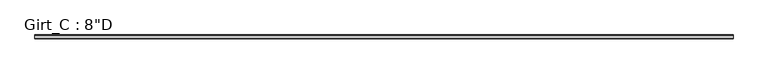
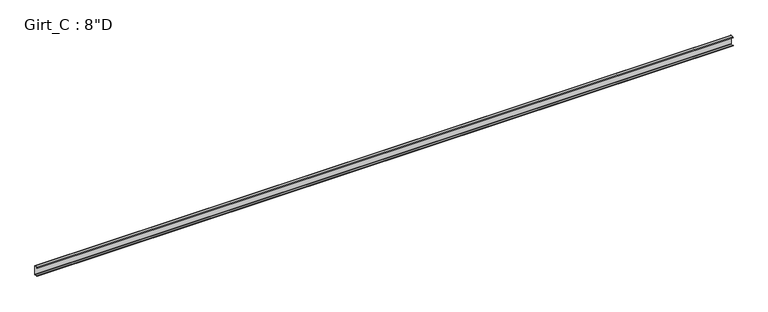
"""IFC4 building model written with IfcOpenShell, lengths in millimetres: beam geometry."""

from ifc_helpers import new_model, si_unit, point, frame, frame_2d, origin, place, context, project, spatial, polyline, circle_curve, trimmed, segment, composite_curve, outline, extrude, source, transform, mapped, element, save


def beam_3230b69d(model_context):
    return source(origin(), model_context, "Body", "SweptSolid", [
        extrude(outline(composite_curve([segment(polyline([(-63.5, 101.6), (-3.3734375, 101.6)]), True, "CONTINUOUS"), segment(trimmed(circle_curve(frame_2d((-3.3734375, 96.8375)), 4.7625), [point((-3.3734375, 101.6))], [point((1.3890625, 96.8375))], False, "CARTESIAN"), True, "CONTINUOUS"), segment(polyline([(1.3890625, 96.8375), (1.3890625, -96.8375)]), True, "CONTINUOUS"), segment(trimmed(circle_curve(frame_2d((-3.3734375, -96.8375)), 4.7625), [point((1.3890625, -96.8375))], [point((-3.3734375, -101.6))], False, "CARTESIAN"), True, "CONTINUOUS"), segment(polyline([(-3.3734375, -101.6), (-63.5, -101.6), (-75.745104, -87.0068534), (-73.6169367, -85.221109), (-62.204539, -98.821875), (-3.2694106, -98.821875)]), True, "CONTINUOUS"), segment(trimmed(circle_curve(frame_2d((-3.3748024, -96.8389339)), 1.9857399), [point((-3.2694106, -98.821875))], [point((-1.3890625, -96.8389339))], True, "CARTESIAN"), True, "CONTINUOUS"), segment(polyline([(-1.3890625, -96.8389339), (-1.3890625, 96.8381931)]), True, "CONTINUOUS"), segment(trimmed(circle_curve(frame_2d((-3.3741066, 96.8381931)), 1.9850441), [point((-1.3890625, 96.8381931))], [point((-3.3005807, 98.821875))], True, "CARTESIAN"), True, "CONTINUOUS"), segment(polyline([(-3.3005807, 98.821875), (-62.204539, 98.821875), (-73.6169367, 85.221109), (-75.745104, 87.0068534), (-63.5, 101.6)]), True, "CONTINUOUS")], self_intersect=False)), frame((-7264.4, 0.0, 0.0), z_axis=(1.0, 0.0, 0.0), x_axis=(0.0, 1.0, 0.0)), (0.0, 0.0, 1.0), 14528.8),
    ])


if __name__ == "__main__":
    model = new_model("IFC4")
    model_context = context("Model", 3, world=origin())
    ifc_project = project(units=[si_unit("LENGTHUNIT", "METRE", prefix="MILLI")], contexts=[model_context])
    site = spatial("IfcSite", under=ifc_project)
    building = spatial("IfcBuilding", under=site)
    placement = place(None, origin())
    beam_shape = beam_3230b69d(model_context)
    element("IfcBeam", 1, ObjectType="Girt_C : 8\"D", at=placement, inside=building, context=model_context, shape_type="MappedRepresentation", body=[
        mapped(beam_shape, transform((0.0, 0.0, 0.0), x_axis=(1.0, 0.0, 0.0), y_axis=(0.0, 1.0, 0.0), z_axis=(0.0, 0.0, 1.0))),
    ])
    save(model, "model.ifc")

# Revit data of these elements
# Type "Girt_C : 8\"D"
#   Web_Thickness = 0' - 0 7/64"
#   Length [instance default] = 10' - 0"
#   Leg_1 = 0' - 2 1/2"
#   Height = 0' - 8"
#   Structural Material [instance default] = none
